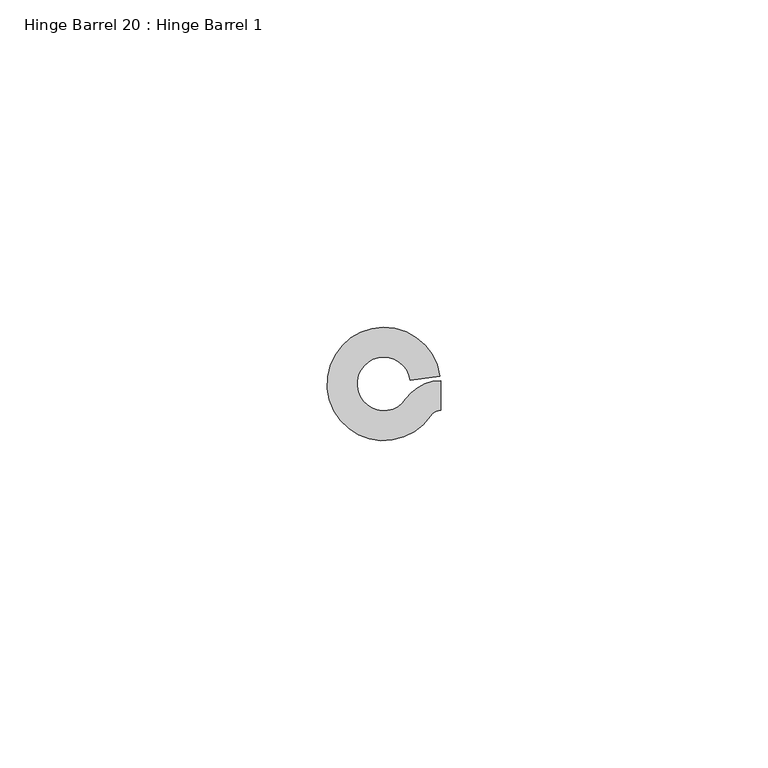
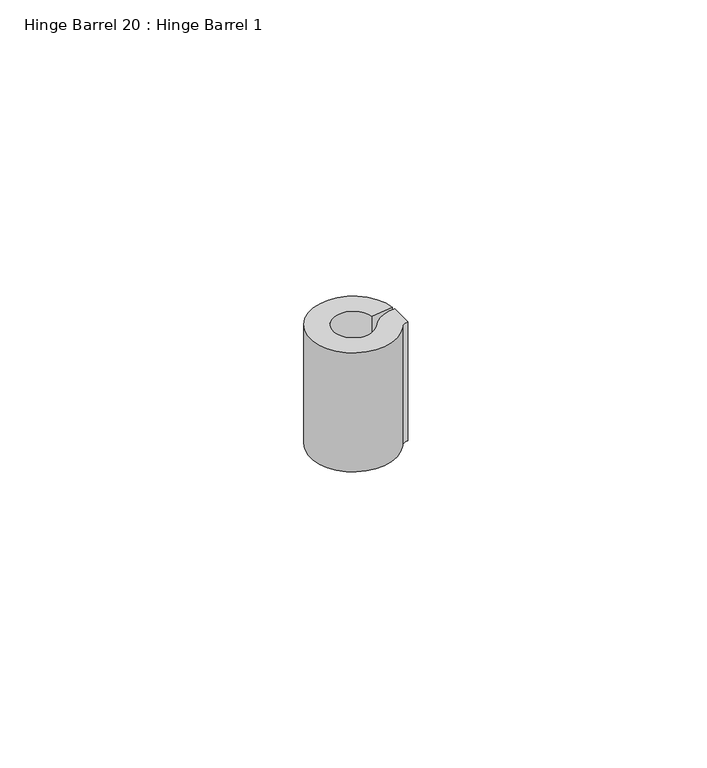
"""IFC4 building model written with IfcOpenShell, lengths in millimetres: proxy geometry, Hinge Barrel 20 : Hinge Barrel 1."""

from ifc_helpers import new_model, si_unit, point, frame, frame_2d, origin, place, context, project, spatial, polyline, circle_curve, trimmed, segment, composite_curve, outline, extrude, source, transform, mapped, element, save


def hinge_barrel_20_hinge_barrel_1_6108b341(model_context):
    return source(origin(), model_context, "Body", "SweptSolid", [
        extrude(outline(composite_curve([segment(trimmed(circle_curve(frame_2d((587327.8245257, -533990.5568067)), 6.4044851), [point((587322.5194669, -533986.9688017))], [point((587327.8245257, -533984.1523216))], False, "CARTESIAN"), True, "CONTINUOUS"), segment(polyline([(587327.8245257, -533984.1523216), (587327.8245257, -533988.7163841)]), True, "CONTINUOUS"), segment(trimmed(circle_curve(frame_2d((587327.8245257, -533990.5568067)), 1.8404226), [point((587327.8245257, -533988.7163841))], [point((587326.3000393, -533989.5257409))], True, "CARTESIAN"), True, "CONTINUOUS"), segment(trimmed(circle_curve(frame_2d((587319.1320739, -533984.6777841)), 8.6534625), [point((587326.3000393, -533989.5257409))], [point((587327.7022899, -533983.4803654))], False, "CARTESIAN"), True, "CONTINUOUS"), segment(polyline([(587327.7022899, -533983.4803654), (587323.1821338, -533984.1119153)]), True, "CONTINUOUS"), segment(trimmed(circle_curve(frame_2d((587319.1320739, -533984.6777841)), 4.0894), [point((587323.1821338, -533984.1119153))], [point((587322.5194669, -533986.9688017))], True, "CARTESIAN"), True, "CONTINUOUS")], self_intersect=False)), frame((0.0, 0.0, 1962.15), z_axis=(0.0, 0.0, 1.0), x_axis=(1.0, 0.0, 0.0)), (0.0, 0.0, 1.0), 25.4),
    ])


if __name__ == "__main__":
    model = new_model("IFC4")
    model_context = context("Model", 3, world=origin())
    ifc_project = project(units=[si_unit("LENGTHUNIT", "METRE", prefix="MILLI")], contexts=[model_context])
    site = spatial("IfcSite", under=ifc_project)
    building = spatial("IfcBuilding", under=site)
    placement = place(None, origin())
    hinge_barrel_20_hinge_barrel_1_shape = hinge_barrel_20_hinge_barrel_1_6108b341(model_context)
    element("IfcBuildingElementProxy", 1, Name="Hinge Barrel 20 : Hinge Barrel 1", ObjectType="Hinge Barrel 20 : Hinge Barrel 1", at=placement, inside=building, context=model_context, shape_type="MappedRepresentation", body=[
        mapped(hinge_barrel_20_hinge_barrel_1_shape, transform((0.0, 0.0, 0.0), x_axis=(1.0, 0.0, 0.0), y_axis=(0.0, 1.0, 0.0), z_axis=(0.0, 0.0, 1.0))),
    ])
    save(model, "model.ifc")

# Revit data of these elements
# Element 1 (IfcBuildingElementProxy, "Hinge Barrel 20 : Hinge Barrel 1")
#   Materials on its faces: "6\"X6\" WELD-ON STL BUTT HINGE"
# Materials
#   "6\"X6\" WELD-ON STL BUTT HINGE": class "Metal", colour RGB 189 187 185, transparency 0, Description = "Carbon steel", Cost = 0
